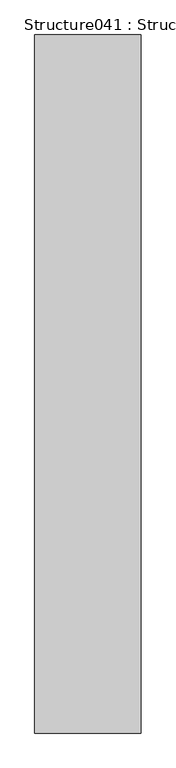
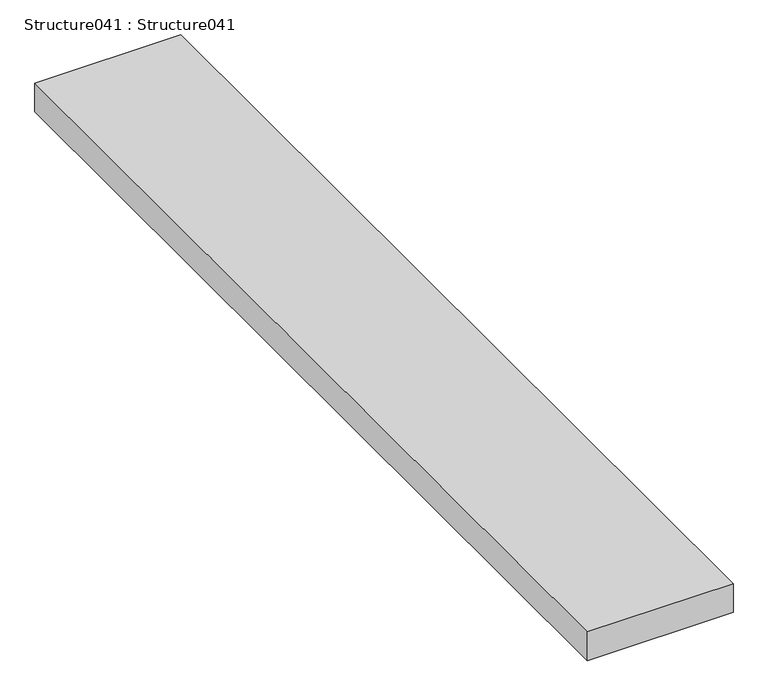
"""IFC4 building model written with IfcOpenShell, lengths in millimetres: proxy geometry, Structure041 : Structure041."""

from ifc_helpers import new_model, si_unit, frame, origin, place, context, project, spatial, polyline, outline, extrude, source, transform, mapped, element, save


def structure041_structure041_46c49756(model_context):
    return source(origin(), model_context, "Body", "SweptSolid", [
        extrude(outline(polyline([(-4682.3338825, -1052.8906574), (-4987.1338825, -1052.8906574), (-4987.1338825, 947.1093426), (-4682.3338825, 947.1093426), (-4682.3338825, -1052.8906574)])), frame((0.0, 0.0, 40049.196), z_axis=(0.0, 0.0, 1.0), x_axis=(1.0, 0.0, 0.0)), (0.0, 0.0, 1.0), 63.5),
    ])


if __name__ == "__main__":
    model = new_model("IFC4")
    model_context = context("Model", 3, world=origin())
    ifc_project = project(units=[si_unit("LENGTHUNIT", "METRE", prefix="MILLI")], contexts=[model_context])
    site = spatial("IfcSite", under=ifc_project)
    building = spatial("IfcBuilding", under=site)
    placement = place(None, origin())
    structure041_structure041_shape = structure041_structure041_46c49756(model_context)
    element("IfcBuildingElementProxy", 1, Name="Structure041 : Structure041", ObjectType="Structure041 : Structure041", at=placement, inside=building, context=model_context, shape_type="MappedRepresentation", body=[
        mapped(structure041_structure041_shape, transform((0.0, 0.0, 0.0), x_axis=(1.0, 0.0, 0.0), y_axis=(0.0, 1.0, 0.0), z_axis=(0.0, 0.0, 1.0))),
    ])
    save(model, "model.ifc")

# Revit data of these elements
# Type "Structure041 : Structure041"
#   NameOverride = "Structure041"
# Element 1 (IfcBuildingElementProxy, "Structure041 : Structure041")
#   Materials on its faces: "STRUCTURAL MEMBER (SEE STRUCTURAL DWGS)"
# Materials
#   "STRUCTURAL MEMBER (SEE STRUCTURAL DWGS)": class "Unassigned", colour RGB 176 134 95, transparency 0, Cost = 0
